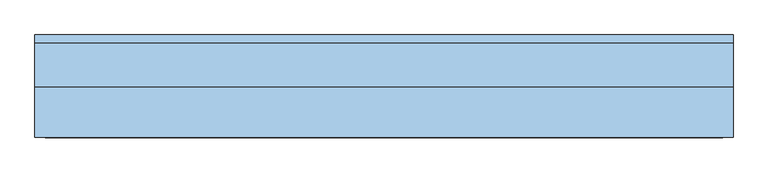
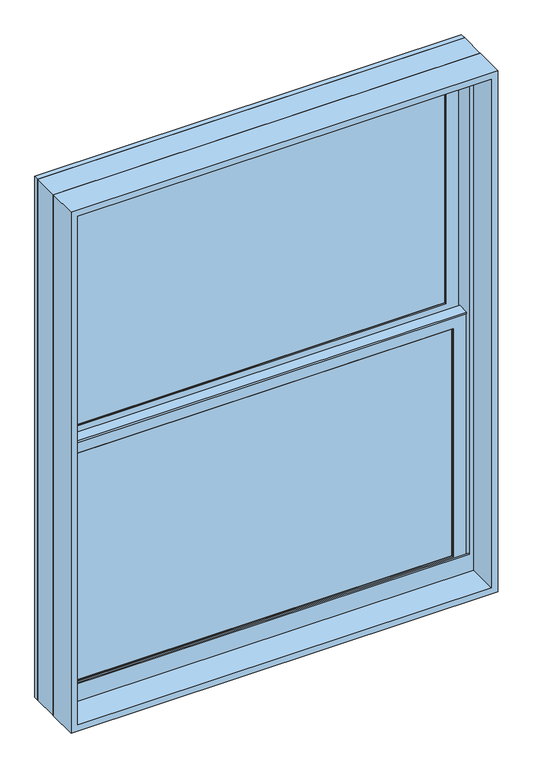
"""IFC4 building model written with IfcOpenShell, lengths in millimetres: window geometry, Window-Double_Hung-Marvin-Essential : ESDH3646."""

from ifc_helpers import new_model, si_unit, frame, origin, place, context, project, spatial, polyline, outline, extrude, faceted_brep, source, transform, mapped, element, save


def window_4eb672f6(model_context):
    return source(origin(), model_context, "Body", "SolidModel", [
        extrude(outline(polyline([(166.1583333, 20.6375), (166.1583333, 15.875), (147.1083333, 15.875), (147.1083333, 20.6375), (166.1583333, 20.6375)])), frame((0.0, 0.0, 1136.65), z_axis=(0.0, 0.0, 1.0), x_axis=(1.0, 0.0, 0.0)), (0.0, 0.0, 1.0), 603.25),
        extrude(outline(polyline([(-147.1083333, 20.6375), (-147.1083333, 15.875), (-166.1583333, 15.875), (-166.1583333, 20.6375), (-147.1083333, 20.6375)])), frame((0.0, 0.0, 1136.65), z_axis=(0.0, 0.0, 1.0), x_axis=(1.0, 0.0, 0.0)), (0.0, 0.0, 1.0), 603.25),
        extrude(outline(polyline([(469.9, 20.6375), (469.9, 15.875), (-469.9, 15.875), (-469.9, 20.6375), (469.9, 20.6375)])), frame((0.0, 0.0, 1428.75), z_axis=(0.0, 0.0, 1.0), x_axis=(1.0, 0.0, 0.0)), (0.0, 0.0, 1.0), 19.05),
        extrude(outline(polyline([(-166.1583333, 46.83125), (-166.1583333, 51.59375), (-147.1083333, 51.59375), (-147.1083333, 46.83125), (-166.1583333, 46.83125)])), frame((0.0, 0.0, 1778.0), z_axis=(0.0, 0.0, 1.0), x_axis=(1.0, 0.0, 0.0)), (0.0, 0.0, 1.0), 603.25),
        extrude(outline(polyline([(147.1083333, 46.83125), (147.1083333, 51.59375), (166.1583333, 51.59375), (166.1583333, 46.83125), (147.1083333, 46.83125)])), frame((0.0, 0.0, 1778.0), z_axis=(0.0, 0.0, 1.0), x_axis=(1.0, 0.0, 0.0)), (0.0, 0.0, 1.0), 603.25),
        extrude(outline(polyline([(-469.9, 46.83125), (-469.9, 51.59375), (469.9, 51.59375), (469.9, 46.83125), (-469.9, 46.83125)])), frame((0.0, 0.0, 2070.1), z_axis=(0.0, 0.0, 1.0), x_axis=(1.0, 0.0, 0.0)), (0.0, 0.0, 1.0), 19.05),
        extrude(outline(polyline([(166.1583333, 20.6375), (147.1083333, 20.6375), (147.1083333, 25.4), (166.1583333, 25.4), (166.1583333, 20.6375)])), frame((0.0, 0.0, 1136.65), z_axis=(0.0, 0.0, 1.0), x_axis=(1.0, 0.0, 0.0)), (0.0, 0.0, 1.0), 603.25),
        extrude(outline(polyline([(-147.1083333, 20.6375), (-166.1583333, 20.6375), (-166.1583333, 25.4), (-147.1083333, 25.4), (-147.1083333, 20.6375)])), frame((0.0, 0.0, 1136.65), z_axis=(0.0, 0.0, 1.0), x_axis=(1.0, 0.0, 0.0)), (0.0, 0.0, 1.0), 603.25),
        extrude(outline(polyline([(469.9, 20.6375), (-469.9, 20.6375), (-469.9, 25.4), (469.9, 25.4), (469.9, 20.6375)])), frame((0.0, 0.0, 1428.75), z_axis=(0.0, 0.0, 1.0), x_axis=(1.0, 0.0, 0.0)), (0.0, 0.0, 1.0), 19.05),
        extrude(outline(polyline([(-166.1583333, 56.35625), (-147.1083333, 56.35625), (-147.1083333, 51.59375), (-166.1583333, 51.59375), (-166.1583333, 56.35625)])), frame((0.0, 0.0, 1778.0), z_axis=(0.0, 0.0, 1.0), x_axis=(1.0, 0.0, 0.0)), (0.0, 0.0, 1.0), 603.25),
        extrude(outline(polyline([(147.1083333, 56.35625), (166.1583333, 56.35625), (166.1583333, 51.59375), (147.1083333, 51.59375), (147.1083333, 56.35625)])), frame((0.0, 0.0, 1778.0), z_axis=(0.0, 0.0, 1.0), x_axis=(1.0, 0.0, 0.0)), (0.0, 0.0, 1.0), 603.25),
        extrude(outline(polyline([(-469.9, 56.35625), (469.9, 56.35625), (469.9, 51.59375), (-469.9, 51.59375), (-469.9, 56.35625)])), frame((0.0, 0.0, 2070.1), z_axis=(0.0, 0.0, 1.0), x_axis=(1.0, 0.0, 0.0)), (0.0, 0.0, 1.0), 19.05),
        faceted_brep([(-496.8875, 5.6780605, 1769.9351748), (-496.8875, 5.6780605, 1765.3), (496.8875, 5.6780605, 1765.3), (496.8875, 5.6780605, 1769.9351748), (-496.8875, 34.8118605, 1769.9351748), (496.8875, 34.8118605, 1769.9351748), (496.8875, 34.8118605, 1765.3), (-496.8875, 34.8118605, 1765.3), (-496.8875, 30.1625, 1765.3), (-496.8875, 30.1625, 1109.6625), (-496.8875, 8.9241104, 1109.6625), (-496.8875, 8.9241104, 1765.3), (496.8875, 8.9241104, 1765.3), (496.8875, 30.1625, 1765.3), (496.8875, 8.9241104, 1109.6625), (496.8875, 30.1625, 1109.6625), (-481.0034752, 11.90625, 1751.0034752), (-481.0034752, 30.1625, 1751.0034752), (481.0034752, 30.1625, 1751.0034752), (481.0034752, 11.90625, 1751.0034752), (-464.34375, 10.4662439, 1734.34375), (-464.34375, 11.90625, 1734.34375), (464.34375, 11.90625, 1734.34375), (464.34375, 10.4662439, 1734.34375), (465.8858834, 8.9241104, 1735.8858834), (-465.8858834, 8.9241104, 1735.8858834), (481.0034752, 30.1625, 1125.5465248), (481.0034752, 11.90625, 1125.5465248), (464.34375, 11.90625, 1142.20625), (464.34375, 10.4662439, 1142.20625), (465.8858834, 8.9241104, 1140.6641166), (-481.0034752, 30.1625, 1125.5465248), (-481.0034752, 11.90625, 1125.5465248), (-464.34375, 11.90625, 1142.20625), (-464.34375, 10.4662439, 1142.20625), (-465.8858834, 8.9241104, 1140.6641166)], [[[0, 1, 2, 3]], [[4, 5, 6, 7]], [[1, 0, 4, 7, 8, 9, 10, 11]], [[2, 1, 11, 12]], [[7, 6, 13, 8]], [[3, 2, 12, 14, 15, 13, 6, 5]], [[0, 3, 5, 4]], [[16, 17, 18, 19]], [[20, 21, 22, 23]], [[20, 23, 24, 25]], [[19, 18, 26, 27]], [[23, 22, 28, 29]], [[24, 23, 29, 30]], [[27, 26, 31, 32]], [[29, 28, 33, 34]], [[30, 29, 34, 35]], [[15, 14, 10, 9]], [[15, 9, 8, 13], [18, 17, 31, 26]], [[17, 16, 32, 31]], [[16, 19, 27, 32], [22, 21, 33, 28]], [[21, 20, 34, 33]], [[20, 25, 35, 34]], [[10, 14, 12, 11], [25, 24, 30, 35]]]),
        extrude(outline(polyline([(38.5955581, 1751.0125), (33.5778968, 1751.0125), (33.5778968, 1752.6), (39.9405976, 1752.6), (39.9405976, 1751.0125), (61.515625, 1751.0125), (47.6307501, 1747.6975159), (38.5955581, 1747.6975159), (38.5955581, 1751.0125)])), frame((-496.8875, 0.0, 0.0), z_axis=(1.0, 0.0, 0.0), x_axis=(0.0, 1.0, 0.0)), (0.0, 0.0, 1.0), 993.775),
        faceted_brep([(527.05, 0.0, 1079.5), (527.05, 0.0, 2438.4), (-527.05, 0.0, 2438.4), (-527.05, 0.0, 1079.5), (500.85625, 0.0, 1140.61875), (-500.85625, 0.0, 1140.61875), (-500.85625, 0.0, 2412.20625), (500.85625, 0.0, 2412.20625), (500.85625, 3.96875, 1079.5), (-500.85625, 3.96875, 1079.5), (-500.85625, 3.96875, 1140.61875), (500.85625, 3.96875, 1140.61875), (-527.05, 65.6828125, 1079.5), (-500.85625, 65.6828125, 1079.5), (500.85625, 65.6828125, 1079.5), (527.05, 65.6828125, 1079.5), (-527.05, 65.6828125, 2438.4), (527.05, 65.6828125, 2438.4), (500.85625, 65.6828125, 2412.20625), (-500.85625, 65.6828125, 2412.20625)], [[[0, 1, 2, 3], [4, 5, 6, 7]], [[8, 9, 10, 11]], [[5, 4, 11, 10]], [[0, 3, 12, 13, 9, 8, 14, 15]], [[13, 12, 16, 17, 15, 14, 18, 19]], [[13, 19, 6, 5, 10, 9]], [[7, 6, 19, 18]], [[18, 14, 8, 11, 4, 7]], [[1, 0, 15, 17]], [[2, 1, 17, 16]], [[3, 2, 16, 12]]]),
        faceted_brep([(500.85625, 30.1625, 1758.95), (499.26875, 30.1625, 1758.95), (499.26875, 30.1625, 1103.8544613), (500.85625, 30.1625, 1103.8544613), (-499.26875, 30.1625, 1758.95), (-500.85625, 30.1625, 1758.95), (-500.85625, 30.1625, 1103.8544613), (-499.26875, 30.1625, 1103.8544613), (499.26875, 63.5, 1758.95), (500.85625, 63.5, 1758.95), (500.85625, 63.5, 1097.3743077), (499.26875, 63.5, 1097.3743077), (-500.85625, 63.5, 1758.95), (-499.26875, 63.5, 1758.95), (-499.26875, 63.5, 1097.3743077), (-500.85625, 63.5, 1097.3743077), (512.1108932, 3.96875, 1108.9460105), (512.1108932, 3.96875, 1079.5), (512.1108932, 65.6828125, 1079.5), (512.1108932, 65.6828125, 1096.950012), (-512.1108932, 3.96875, 1079.5), (-512.1108932, 3.96875, 1108.9460105), (-512.1108932, 65.6828125, 1096.950012), (-512.1108932, 65.6828125, 1079.5), (512.1108932, 78.58125, 1094.4428097), (-512.1108932, 78.58125, 1094.4428097), (-510.0971252, 68.2348864, 1096.4539391), (-492.13135, 68.2348864, 1096.4539391), (-492.13135, 65.6828125, 1096.950012), (492.13135, 65.6828125, 1096.950012), (492.13135, 68.2348864, 1096.4539391), (510.0971252, 68.2348864, 1096.4539391), (-527.05, 65.6828125, 1079.5), (-527.05, 78.5948249, 1079.5), (527.05, 78.5948249, 1079.5), (527.05, 65.6828125, 1079.5), (-527.05, 78.58125, 2438.4), (527.05, 78.58125, 2438.4), (512.1108932, 78.58125, 2423.4608932), (-512.1108932, 78.58125, 2423.4608932), (-527.05, 65.6828125, 2438.4), (-510.0971252, 68.2348864, 2421.4471252), (510.0971252, 68.2348864, 2421.4471252), (492.13135, 68.2348864, 2403.48135), (-492.13135, 68.2348864, 2403.48135), (-492.13135, 65.6828125, 2403.48135), (492.13135, 65.6828125, 2403.48135), (527.05, 65.6828125, 2438.4)], [[[0, 1, 2, 3]], [[4, 5, 6, 7]], [[8, 9, 10, 11]], [[12, 13, 14, 15]], [[1, 8, 11, 2]], [[9, 0, 3, 10]], [[1, 0, 9, 8]], [[5, 4, 13, 12]], [[5, 12, 15, 6]], [[13, 4, 7, 14]], [[16, 17, 18, 19]], [[20, 21, 22, 23]], [[24, 25, 26, 27, 28, 22, 21, 16, 19, 29, 30, 31], [3, 2, 11, 10], [7, 6, 15, 14]], [[17, 16, 21, 20]], [[17, 20, 23, 32, 33, 34, 35, 18]], [[34, 33, 36, 37], [25, 24, 38, 39]], [[33, 32, 40, 36]], [[39, 41, 26, 25]], [[41, 42, 31, 30, 43, 44, 27, 26]], [[44, 45, 28, 27]], [[40, 32, 23, 22, 28, 45, 46, 29, 19, 18, 35, 47]], [[36, 40, 47, 37]], [[39, 38, 42, 41]], [[44, 43, 46, 45]], [[34, 37, 47, 35]], [[42, 38, 24, 31]], [[46, 43, 30, 29]]]),
        extrude(outline(polyline([(477.04375, 11.90625), (-477.04375, 11.90625), (-477.04375, 15.08125), (477.04375, 15.08125), (477.04375, 11.90625)])), frame((0.0, 0.0, 1129.50625), z_axis=(0.0, 0.0, 1.0), x_axis=(1.0, 0.0, 0.0)), (0.0, 0.0, 1.0), 617.5375),
        extrude(outline(polyline([(477.04375, 42.8625), (-477.04375, 42.8625), (-477.04375, 46.0375), (477.04375, 46.0375), (477.04375, 42.8625)])), frame((0.0, 0.0, 1770.85625), z_axis=(0.0, 0.0, 1.0), x_axis=(1.0, 0.0, 0.0)), (0.0, 0.0, 1.0), 617.5375),
        faceted_brep([(-464.34375, 31.194477, 1734.34375), (-465.8858834, 32.7366104, 1735.8858834), (465.8858834, 32.7366104, 1735.8858834), (464.34375, 31.194477, 1734.34375), (-464.34375, 30.1625, 1734.34375), (464.34375, 30.1625, 1734.34375), (-496.8875, 32.7366104, 1766.8875), (-496.8875, 30.1625, 1766.8875), (496.8875, 30.1625, 1766.8875), (496.8875, 32.7366104, 1766.8875), (465.8858834, 32.7366104, 1140.6641166), (464.34375, 31.194477, 1142.20625), (464.34375, 30.1625, 1142.20625), (496.8875, 30.1625, 1109.6625), (496.8875, 32.7366104, 1109.6625), (-465.8858834, 32.7366104, 1140.6641166), (-464.34375, 31.194477, 1142.20625), (-464.34375, 30.1625, 1142.20625), (-496.8875, 30.1625, 1109.6625), (-496.8875, 32.7366104, 1109.6625)], [[[0, 1, 2, 3]], [[4, 0, 3, 5]], [[6, 7, 8, 9]], [[3, 2, 10, 11]], [[5, 3, 11, 12]], [[9, 8, 13, 14]], [[11, 10, 15, 16]], [[12, 11, 16, 17]], [[14, 13, 18, 19]], [[9, 14, 19, 6], [1, 15, 10, 2]], [[16, 15, 1, 0]], [[17, 16, 0, 4]], [[7, 18, 13, 8], [5, 12, 17, 4]], [[19, 18, 7, 6]]]),
        faceted_brep([(-481.0034752, 42.8625, 2392.3534752), (-481.0034752, 61.11875, 2392.3534752), (481.0034752, 61.11875, 2392.3534752), (481.0034752, 42.8625, 2392.3534752), (-464.34375, 41.4224939, 2375.69375), (-464.34375, 42.8625, 2375.69375), (464.34375, 42.8625, 2375.69375), (464.34375, 41.4224939, 2375.69375), (-465.8858834, 39.8803604, 2377.2358834), (465.8858834, 39.8803604, 2377.2358834), (-496.8875, 61.11875, 2408.2375), (-496.8875, 39.8803604, 2408.2375), (496.8875, 39.8803604, 2408.2375), (496.8875, 61.11875, 2408.2375), (481.0034752, 61.11875, 1766.8965248), (481.0034752, 42.8625, 1766.8965248), (464.34375, 42.8625, 1783.55625), (464.34375, 41.4224939, 1783.55625), (465.8858834, 39.8803604, 1782.0141166), (496.8875, 39.8803604, 1751.0125), (496.8875, 61.11875, 1751.0125), (-481.0034752, 61.11875, 1766.8965248), (-481.0034752, 42.8625, 1766.8965248), (-464.34375, 42.8625, 1783.55625), (-464.34375, 41.4224939, 1783.55625), (-465.8858834, 39.8803604, 1782.0141166), (-496.8875, 39.8803604, 1751.0125), (-496.8875, 61.11875, 1751.0125)], [[[0, 1, 2, 3]], [[4, 5, 6, 7]], [[8, 4, 7, 9]], [[10, 11, 12, 13]], [[3, 2, 14, 15]], [[7, 6, 16, 17]], [[9, 7, 17, 18]], [[13, 12, 19, 20]], [[15, 14, 21, 22]], [[17, 16, 23, 24]], [[18, 17, 24, 25]], [[20, 19, 26, 27]], [[13, 20, 27, 10], [1, 21, 14, 2]], [[22, 21, 1, 0]], [[3, 15, 22, 0], [5, 23, 16, 6]], [[24, 23, 5, 4]], [[25, 24, 4, 8]], [[11, 26, 19, 12], [9, 18, 25, 8]], [[27, 26, 11, 10]]]),
        faceted_brep([(-496.8875, 61.11875, 1751.0125), (-496.8875, 63.6928604, 1751.0125), (496.8875, 63.6928604, 1751.0125), (496.8875, 61.11875, 1751.0125), (-464.34375, 62.150727, 1783.55625), (-464.34375, 61.11875, 1783.55625), (464.34375, 61.11875, 1783.55625), (464.34375, 62.150727, 1783.55625), (-465.8858834, 63.6928604, 1782.0141166), (465.8858834, 63.6928604, 1782.0141166), (496.8875, 63.6928604, 2408.2375), (496.8875, 61.11875, 2408.2375), (464.34375, 61.11875, 2375.69375), (464.34375, 62.150727, 2375.69375), (465.8858834, 63.6928604, 2377.2358834), (-496.8875, 63.6928604, 2408.2375), (-496.8875, 61.11875, 2408.2375), (-464.34375, 61.11875, 2375.69375), (-464.34375, 62.150727, 2375.69375), (-465.8858834, 63.6928604, 2377.2358834)], [[[0, 1, 2, 3]], [[4, 5, 6, 7]], [[8, 4, 7, 9]], [[3, 2, 10, 11]], [[7, 6, 12, 13]], [[9, 7, 13, 14]], [[11, 10, 15, 16]], [[13, 12, 17, 18]], [[14, 13, 18, 19]], [[16, 15, 1, 0]], [[3, 11, 16, 0], [5, 17, 12, 6]], [[18, 17, 5, 4]], [[19, 18, 4, 8]], [[1, 15, 10, 2], [9, 14, 19, 8]]]),
        extrude(outline(polyline([(477.04375, 26.19375), (-477.04375, 26.19375), (-477.04375, 30.1625), (477.04375, 30.1625), (477.04375, 26.19375)])), frame((0.0, 0.0, 1129.50625), z_axis=(0.0, 0.0, 1.0), x_axis=(1.0, 0.0, 0.0)), (0.0, 0.0, 1.0), 617.5375),
        extrude(outline(polyline([(477.04375, 57.15), (-477.04375, 57.15), (-477.04375, 61.11875), (477.04375, 61.11875), (477.04375, 57.15)])), frame((0.0, 0.0, 1770.85625), z_axis=(0.0, 0.0, 1.0), x_axis=(1.0, 0.0, 0.0)), (0.0, 0.0, 1.0), 617.5375),
        extrude(outline(polyline([(2438.4, 527.05), (2438.4, -527.05), (1079.5, -527.05), (1079.5, 527.05), (2438.4, 527.05)]), holes=[polyline([(2422.525, 511.175), (1095.375, 511.175), (1095.375, -511.175), (2422.525, -511.175), (2422.525, 511.175)])]), frame((0.0, -76.2, 0.0), z_axis=(0.0, 1.0, 0.0), x_axis=(0.0, 0.0, 1.0)), (0.0, 0.0, 1.0), 75.40625),
    ])


if __name__ == "__main__":
    model = new_model("IFC4")
    model_context = context("Model", 3, world=origin())
    ifc_project = project(units=[si_unit("LENGTHUNIT", "METRE", prefix="MILLI")], contexts=[model_context])
    site = spatial("IfcSite", under=ifc_project)
    building = spatial("IfcBuilding", under=site)
    placement = place(None, origin())
    window_shape = window_4eb672f6(model_context)
    element("IfcWindow", 1, ObjectType="Window-Double_Hung-Marvin-Essential : ESDH3646", at=placement, inside=building, context=model_context, shape_type="MappedRepresentation", body=[
        mapped(window_shape, transform((0.0, 0.0, 0.0), x_axis=(1.0, 0.0, 0.0), y_axis=(0.0, 1.0, 0.0), z_axis=(0.0, 0.0, 1.0))),
    ])
    save(model, "model.ifc")

# Revit data of these elements
# Type "Window-Double_Hung-Marvin-Essential : ESDH3646"
#   Type Mark = "59"
#   Window Type = "Essential Double Hung"
#   Product data url = "https://bimobject.com/marvin-windows-and-doors/product/marvin-dhwau"
#   Product Guid = "c4a96547-874c-4385-91dc-a058adc19d98"
#   Frame = "All Ultrex"
#   Egress Window = "No"
#   URL = "www.marvin.com"
#   Model = "ESDH3646"
#   Manufacturer = "Marvin Windows and Doors"
#   Label Egress = ""
#   Glass Type = "IG Low E II with Argon"
#   Design Pressure = "DP40"
#   Description = "4254 DBHG"
#   Analytic Construction = "<None>"
#   Prairie Corner Width = 0' - 4"
#   Prairie Corner Height = 0' - 4"
#   Egress Width = 3' - 2 9/16"
#   Egress Height = 1' - 10 27/128"
#   Rough Width = 3' - 6"
#   Rough Height = 4' - 6"
#   Nominal Width = 3' - 6"
#   Nominal Height = 4' - 6"
#   Inset to Installation Flange [instance default] = 0' - 1"
#   Height = 4' - 5 1/2"
#   Egress Area = 5.94798 SF
#   Default Head Height = 8' - 0"
#   Width = 3' - 5 1/2"
#   Daylight Area = 11.8384 SF
#   DLO Width = 3' - 0 9/16"
#   DLO Height = 1' - 11 5/16"
#   Muntins Top Sash = yes
#   Lites Wide Top Sash = 3
#   Lites Wide Bottom Sash = 3
#   Lites High Top Sash = 2
#   Lites High Bottom Sash = 2
#   Lite Cut Prairie 9 = no
#   Lite Cut HV Grid = yes
#   Muntins Bottom Sash = yes
#   Label Visibility = no
#   Jamb Extension Visibility = yes
#   Edition number = 1
#   Interior Material = Ultrex-Marvin-Stonewhite
#   Glazing Material = Glass-Marvin-IG Low E II with Argon
#   Cladding Material = Ultrex-Marvin-Pebblegray
#   Wall Closure = (empty or 0)
#   Assembly Code = ""
# Element 1 (IfcWindow, "Window-Double_Hung-Marvin-Essential : ESDH3646")
#   Materials on its faces: "Ultrex-Marvin-Pebblegray", "Ultrex-Marvin-Stonewhite", "Glass-Marvin-IG Low E II with Argon"
# Materials
#   "Ultrex-Marvin-Stonewhite": class "Paint", colour RGB 250 251 245, transparency 0
#   "Glass-Marvin-IG Low E II with Argon": class "Glass", colour RGB 0 128 192, transparency 0.85
#   "Ultrex-Marvin-Pebblegray": class "Paint", colour RGB 189 185 173, transparency 0
